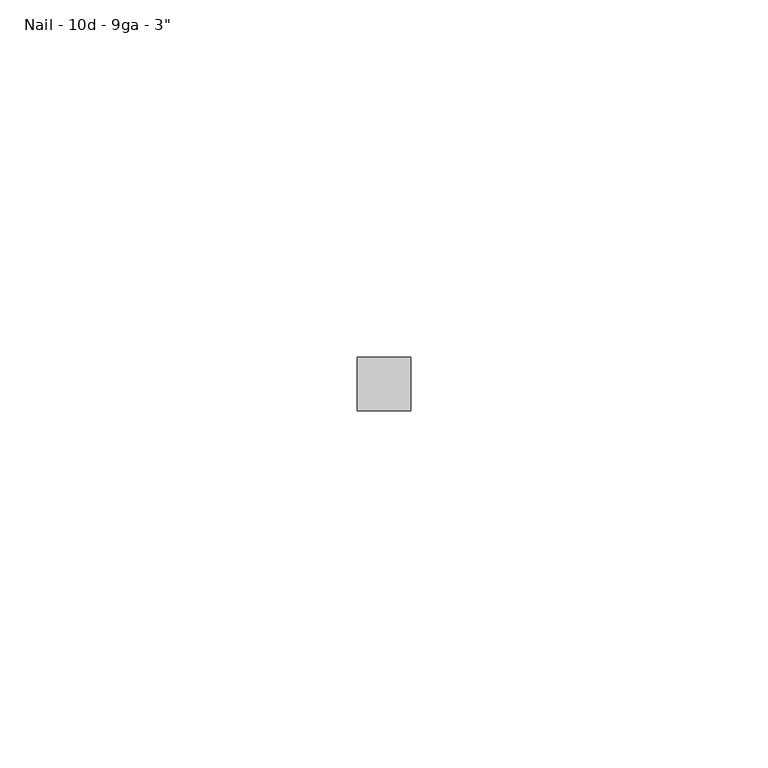
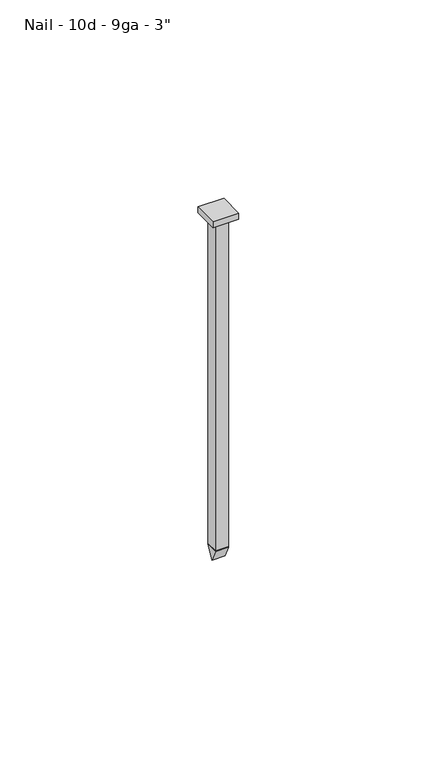
"""IFC4 building model written with IfcOpenShell, lengths in millimetres: fastener geometry."""

from ifc_helpers import new_model, si_unit, frame, origin, origin_with_axes, place, context, project, spatial, polyline, outline, extrude, source, transform, mapped, element, save


def fastener_f1a54bc9(model_context):
    return source(origin(), model_context, "Body", "SweptSolid", [
        extrude(outline(polyline([(0.0, -105.3592), (-1.8796, -101.6), (1.8796, -101.6), (0.0, -105.3592)])), frame((-1.8796, 0.0, 0.0), z_axis=(1.0, 0.0, 0.0), x_axis=(0.0, 1.0, 0.0)), (0.0, 0.0, 1.0), 3.7592),
        extrude(outline(polyline([(-3.7592, -3.7592), (-3.7592, 3.7592), (3.7592, 3.7592), (3.7592, -3.7592), (-3.7592, -3.7592)])), origin_with_axes(), (0.0, 0.0, 1.0), 1.8796),
        extrude(outline(polyline([(-1.8796, 1.8796), (1.8796, 1.8796), (1.8796, -1.8796), (-1.8796, -1.8796), (-1.8796, 1.8796)])), frame((0.0, 0.0, -101.6), z_axis=(0.0, 0.0, 1.0), x_axis=(1.0, 0.0, 0.0)), (0.0, 0.0, 1.0), 101.6),
    ])


if __name__ == "__main__":
    model = new_model("IFC4")
    model_context = context("Model", 3, world=origin())
    ifc_project = project(units=[si_unit("LENGTHUNIT", "METRE", prefix="MILLI")], contexts=[model_context])
    site = spatial("IfcSite", under=ifc_project)
    building = spatial("IfcBuilding", under=site)
    placement = place(None, origin())
    fastener_shape = fastener_f1a54bc9(model_context)
    element("IfcFastener", 1, ObjectType="060523 - W_P_C - Fastenings - Generic - SQUARE : Nail - 10d - 9ga - 3\"", at=placement, inside=building, context=model_context, shape_type="MappedRepresentation", body=[
        mapped(fastener_shape, transform((0.0, 0.0, 0.0), x_axis=(1.0, 0.0, 0.0), y_axis=(0.0, 1.0, 0.0), z_axis=(0.0, 0.0, 1.0))),
    ])
    save(model, "model.ifc")

# Revit data of these elements
# Type "060523 - W_P_C - Fastenings - Generic - SQUARE : Nail - 10d - 9ga - 3\""
#   Washer_Thickness = 0' - 0.00333"
#   Washer Radius = 0' - 0.084"
#   Washer Offset - Head = 0' - 0"
#   Washer Offset = 0' - 0"
#   Thickness_of_Substrate [instance default] = 0' - 1"
#   Side = 0' - 0 37/64"
#   Radius = 0' - 0.074"
#   Length [instance default] = 0' - 3"
#   Head Size = 0' - 1"
#   Head Radius = 0' - 0 1/2"
#   Head Height = 0' - 0.01"
#   Double Diameter = 0' - 0.296"
#   Diameter = 0' - 0.148"
#   Default Elevation = 4' - 0"
#   Washer_Nut_Visibility = no
#   Washer_Head_Visibility = no
#   Round_Head_Visibility = yes
#   Point Visibility = yes
#   Nut_Visibility = no
#   Hex_Head_Visiblilty = no
#   Washer Material = none
#   Bolt Material (Size) = AT SILL - FASTENER AT 24" O.C.
# Element 1 (IfcFastener, "060523 - W_P_C - Fastenings - Generic - SQUARE : Nail - 10d - 9ga - 3\"")
#   Length = 0' - 4"
# Materials
#   "AT SILL - FASTENER AT 24\" O.C.": class "Generic", colour RGB 120 120 120, transparency 0, Cost = 0
